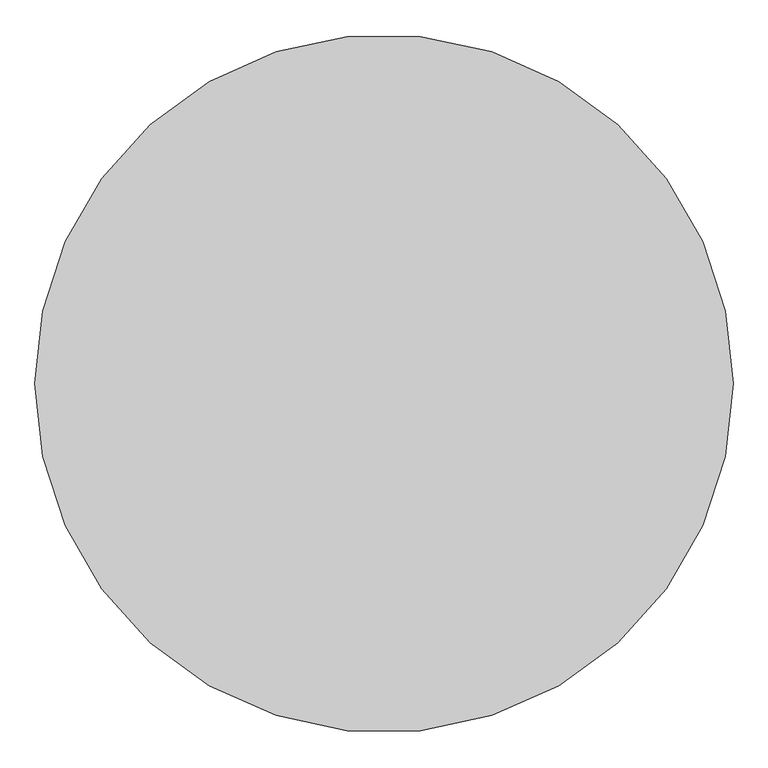
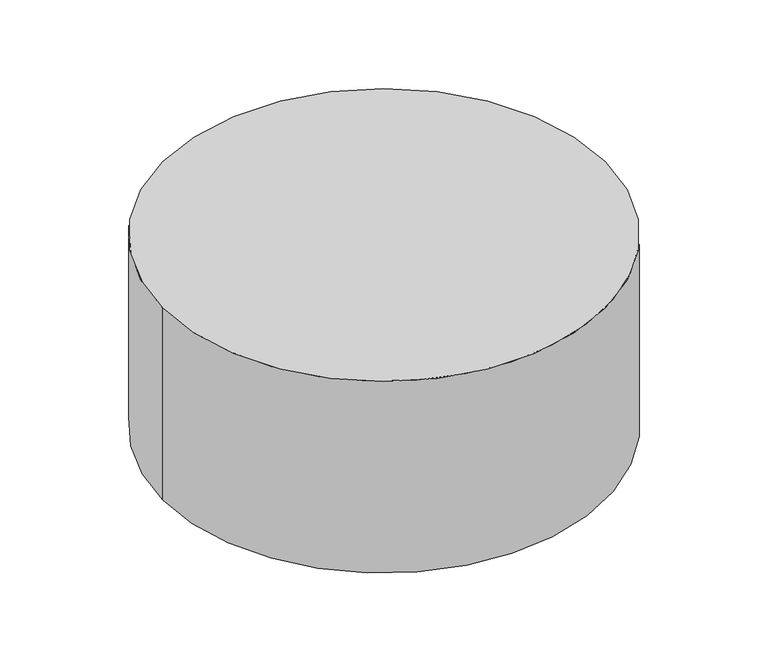
"""IFC4 building model written with IfcOpenShell, lengths in millimetres: proxy geometry, 일반 모델 1 : 일반 모델 1."""

from ifc_helpers import new_model, si_unit, point, frame, frame_2d, origin, place, context, project, spatial, circle_curve, trimmed, segment, composite_curve, outline, extrude, source, transform, mapped, element, save


def generic_models_730128c5(model_context):
    return source(origin(), model_context, "Body", "SweptSolid", [
        extrude(outline(composite_curve([segment(trimmed(circle_curve(frame_2d((-7311.0846298, 1686.0787599)), 1200.0), [point((-8511.0846298, 1686.0787599))], [point((-6111.0846298, 1686.0787599))], False, "CARTESIAN"), True, "CONTINUOUS"), segment(trimmed(circle_curve(frame_2d((-7311.0846298, 1686.0787599)), 1200.0), [point((-6111.0846298, 1686.0787599))], [point((-8511.0846298, 1686.0787599))], False, "CARTESIAN"), True, "CONTINUOUS")], self_intersect=False)), frame((0.0, 0.0, 250.0), z_axis=(0.0, 0.0, 1.0), x_axis=(1.0, 0.0, 0.0)), (0.0, 0.0, 1.0), 1100.0),
    ])


if __name__ == "__main__":
    model = new_model("IFC4")
    model_context = context("Model", 3, world=origin())
    ifc_project = project(units=[si_unit("LENGTHUNIT", "METRE", prefix="MILLI")], contexts=[model_context])
    site = spatial("IfcSite", under=ifc_project)
    building = spatial("IfcBuilding", under=site)
    placement = place(None, origin())
    generic_models_shape = generic_models_730128c5(model_context)
    element("IfcBuildingElementProxy", 1, Name="일반 모델 1 : 일반 모델 1", ObjectType="일반 모델 1 : 일반 모델 1", at=placement, inside=building, context=model_context, shape_type="MappedRepresentation", body=[
        mapped(generic_models_shape, transform((0.0, 0.0, 0.0), x_axis=(1.0, 0.0, 0.0), y_axis=(0.0, 1.0, 0.0), z_axis=(0.0, 0.0, 1.0))),
    ])
    save(model, "model.ifc")

# Revit data of these elements
# Project information
#   프로젝트 발행 날짜 = "발행 날짜"
#   프로젝트 상태 = "프로젝트 상태"
#   클라이언트 이름 = "소유자"
#   프로젝트 주소 = "주소를 여기에 입력"
#   프로젝트 이름 = "프로젝트 이름"
#   프로젝트 번호 = "프로젝트 번호"
# Type "일반 모델 1 : 일반 모델 1"
#   Type Mark = "StepLED.L.B.1"
# Element 1 (IfcBuildingElementProxy, "일반 모델 1 : 일반 모델 1")
#   Materials on its faces: "led_r"
# Materials
#   "led_r": class "일반", colour RGB 255 0 0, transparency 1, Cost = 0
